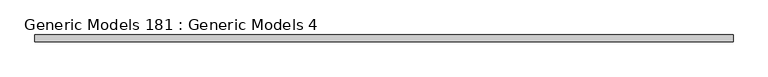
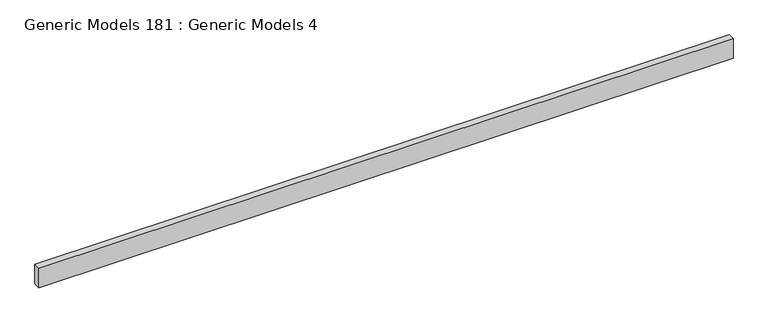
"""IFC4 building model written with IfcOpenShell, lengths in millimetres: proxy geometry, Generic Models 181 : Generic Models 4."""

from ifc_helpers import new_model, si_unit, frame, origin, place, context, project, spatial, polyline, outline, extrude, source, transform, mapped, element, save


def generic_models_181_generic_models_4_5d2d5636(model_context):
    return source(origin(), model_context, "Body", "SweptSolid", [
        extrude(outline(polyline([(2196.9263704, -5316.6308306), (2196.9263704, -5440.4558306), (-10256.7421316, -5440.4558306), (-10256.7421316, -5316.6308306), (2196.9263704, -5316.6308306)])), frame((0.0, 0.0, 126027.7280113), z_axis=(0.0, 0.0, 1.0), x_axis=(1.0, 0.0, 0.0)), (0.0, 0.0, 1.0), 368.7679887),
    ])


if __name__ == "__main__":
    model = new_model("IFC4")
    model_context = context("Model", 3, world=origin())
    ifc_project = project(units=[si_unit("LENGTHUNIT", "METRE", prefix="MILLI")], contexts=[model_context])
    site = spatial("IfcSite", under=ifc_project)
    building = spatial("IfcBuilding", under=site)
    placement = place(None, origin())
    generic_models_181_generic_models_4_shape = generic_models_181_generic_models_4_5d2d5636(model_context)
    element("IfcBuildingElementProxy", 1, Name="Generic Models 181 : Generic Models 4", ObjectType="Generic Models 181 : Generic Models 4", at=placement, inside=building, context=model_context, shape_type="MappedRepresentation", body=[
        mapped(generic_models_181_generic_models_4_shape, transform((0.0, 0.0, 0.0), x_axis=(1.0, 0.0, 0.0), y_axis=(0.0, 1.0, 0.0), z_axis=(0.0, 0.0, 1.0))),
    ])
    save(model, "model.ifc")

# Revit data of these elements
# Element 1 (IfcBuildingElementProxy, "Generic Models 181 : Generic Models 4")
#   Materials on its faces: "_BATT INSUL. (U-FACTOR = 0.065 MIN.) OVER CLASS II VAPOR RETARDER(TOWARD INTERIOR)"
# Materials
#   "_BATT INSUL. (U-FACTOR = 0.065 MIN.) OVER CLASS II VAPOR RETARDER(TOWARD INTERIOR)": class "Generic", colour RGB 227 210 251, transparency 0, Cost = 0
